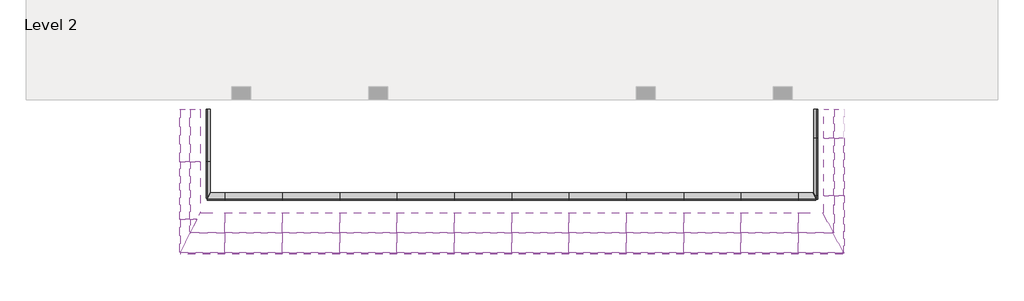
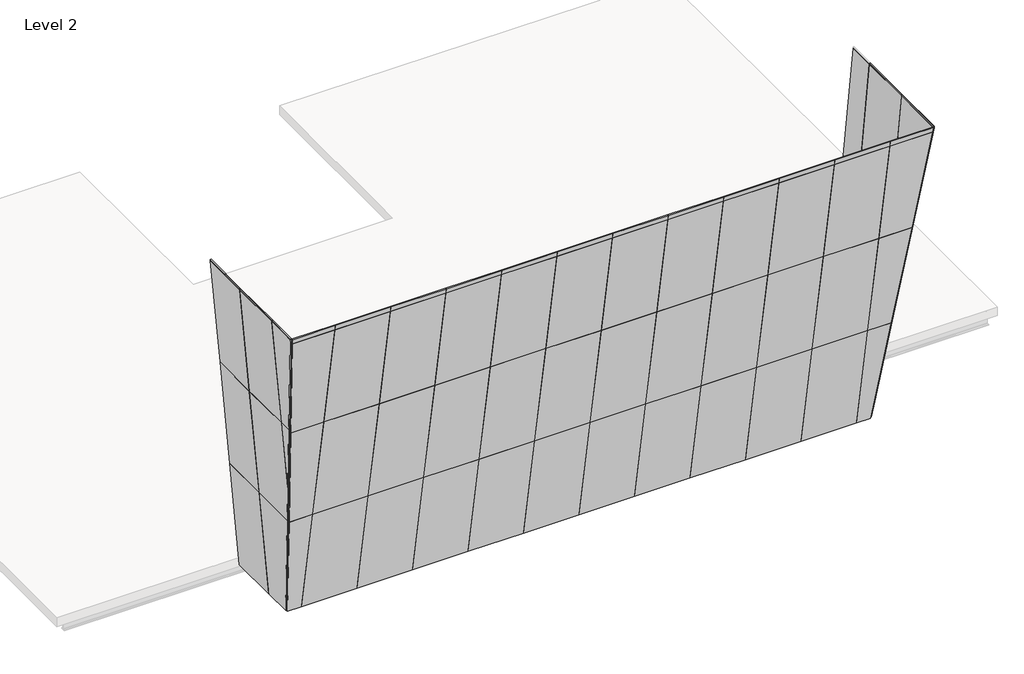
# One storey, part 1 of 2: 70 plates.
"""IFC4 building model written with IfcOpenShell, lengths in millimetres."""

import ifcopenshell
import ifcopenshell.guid

model = None  # the IFC model being written
_history = None  # IfcOwnerHistory: only IFC2X3 demands one
_inside = {}  # id of a spatial element -> (the spatial element, [elements in it])
_under = {}  # id of a project, library or spatial element -> (it, [spatial elements below it])
_declared = {}  # id of a project -> (the project, [libraries it declares])
_typed = {}  # id of a type object -> (the type object, [elements of that type])
_made_of = {}  # id of a material, layer set ... -> (it, [elements and type objects made of it])


def new_model(schema):
    """Start an empty IFC model of exactly this schema.

    Asked for "IFC4X3", IfcOpenShell would pick the latest addendum, in which some entities
    have other attributes; the version numbers below select the first issue.
    IFC2X3 requires an IfcOwnerHistory on every rooted entity: one is made here for all.
    """
    global model, _history
    if schema == "IFC4X3":
        model = ifcopenshell.file(schema_version=(4, 3, 0, 0))
    else:
        model = ifcopenshell.file(schema=schema)
    _inside.clear()
    _under.clear()
    _declared.clear()
    _typed.clear()
    _made_of.clear()
    _history = None
    if model.schema == "IFC2X3":
        org = make("IfcOrganization", Name="unknown")
        user = make(
            "IfcPersonAndOrganization",
            ThePerson=make("IfcPerson", FamilyName="unknown"),
            TheOrganization=org,
        )
        app = make(
            "IfcApplication",
            ApplicationDeveloper=org,
            Version="unknown",
            ApplicationFullName="unknown",
            ApplicationIdentifier="unknown",
        )
        _history = make(
            "IfcOwnerHistory",
            OwningUser=user,
            OwningApplication=app,
            ChangeAction="ADDED",
            CreationDate=0,
        )
    return model


def make(cls, **values):
    """One entity of the class cls with the attributes given. An attribute that is None is left unset."""
    return model.create_entity(
        cls, **{name: value for name, value in values.items() if value is not None}
    )


def rooted(cls, **values):
    """An entity with a GlobalId (a new one), such as an element, a storey or a relation."""
    return make(cls, GlobalId=ifcopenshell.guid.new(), OwnerHistory=_history, **values)


def si_unit(unit_type, name, prefix=None):
    """IfcSIUnit, for example si_unit("LENGTHUNIT", "METRE", prefix="MILLI")."""
    return make("IfcSIUnit", UnitType=unit_type, Prefix=prefix, Name=name)


def assignment(units):
    """IfcUnitAssignment: the units of a project."""
    return None if units is None else make("IfcUnitAssignment", Units=units)


def point(xyz):
    """IfcCartesianPoint."""
    return None if xyz is None else make("IfcCartesianPoint", Coordinates=xyz)


def direction(xyz):
    """IfcDirection."""
    return None if xyz is None else make("IfcDirection", DirectionRatios=xyz)


def frame(location, z_axis=None, x_axis=None):
    """IfcAxis2Placement3D, a coordinate frame: its origin and axes. An axis left out is left unset."""
    return make(
        "IfcAxis2Placement3D",
        Location=point(location),
        Axis=direction(z_axis),
        RefDirection=direction(x_axis),
    )


def origin():
    """The frame at (0, 0, 0) with its axes left unset."""
    return frame((0.0, 0.0, 0.0))


def origin_with_axes():
    """The frame at (0, 0, 0) with the z axis (0, 0, 1) and the x axis (1, 0, 0) written out."""
    return frame((0.0, 0.0, 0.0), z_axis=(0.0, 0.0, 1.0), x_axis=(1.0, 0.0, 0.0))


def place(relative_to, where):
    """IfcLocalPlacement: puts the frame where relative to a parent placement (None: the world)."""
    return make(
        "IfcLocalPlacement", PlacementRelTo=relative_to, RelativePlacement=where
    )


def context(
    kind, dimensions, precision=None, world=None, true_north=None, identifier=None
):
    """IfcGeometricRepresentationContext, for example the 3D "Model" context."""
    return make(
        "IfcGeometricRepresentationContext",
        ContextIdentifier=identifier,
        ContextType=kind,
        CoordinateSpaceDimension=dimensions,
        Precision=precision,
        WorldCoordinateSystem=world,
        TrueNorth=true_north,
    )


def project(units=None, contexts=None):
    """IfcProject with its units and contexts."""
    return rooted(
        "IfcProject",
        Name="project",
        RepresentationContexts=contexts,
        UnitsInContext=assignment(units),
    )


def spatial(cls, under=None, at=None, **own):
    """A site, building, storey or space (cls), placed at a placement, below another one or the project."""
    s = rooted(cls, ObjectPlacement=at, **own)
    if under is not None:
        _under.setdefault(under.id(), (under, []))[1].append(s)
    return s


def polyline(points):
    """IfcPolyline through the points."""
    return make("IfcPolyline", Points=[point(p) for p in points])


def outline(outer, holes=None, kind="AREA"):
    """IfcArbitraryClosedProfileDef: a profile drawn as a closed curve; with holes, ...WithVoids."""
    if holes is None:
        return make("IfcArbitraryClosedProfileDef", ProfileType=kind, OuterCurve=outer)
    return make(
        "IfcArbitraryProfileDefWithVoids",
        ProfileType=kind,
        OuterCurve=outer,
        InnerCurves=holes,
    )


def extrude(swept, where, along, depth):
    """IfcExtrudedAreaSolid: the profile swept, set in the frame where, extruded along a direction by depth."""
    return make(
        "IfcExtrudedAreaSolid",
        SweptArea=swept,
        Position=where,
        ExtrudedDirection=direction(along),
        Depth=depth,
    )


def shape(context_of_items, identifier, shape_type, items):
    """IfcShapeRepresentation: the items that make up one representation, for example the "Body"."""
    return make(
        "IfcShapeRepresentation",
        ContextOfItems=context_of_items,
        RepresentationIdentifier=identifier,
        RepresentationType=shape_type,
        Items=items,
    )


def source(mapping_origin, context_of_items, identifier, shape_type, items):
    """IfcRepresentationMap: a shape defined once, which mapped items show again and again."""
    return make(
        "IfcRepresentationMap",
        MappingOrigin=mapping_origin,
        MappedRepresentation=shape(context_of_items, identifier, shape_type, items),
    )


def transform(
    local_origin,
    x_axis=None,
    y_axis=None,
    z_axis=None,
    scale=None,
    scale2=None,
    scale3=None,
    uniform=True,
):
    """IfcCartesianTransformationOperator3D, or its non-uniform kind. x_axis, y_axis, z_axis: its Axis1, 2, 3."""
    if uniform:
        return make(
            "IfcCartesianTransformationOperator3D",
            Axis1=direction(x_axis),
            Axis2=direction(y_axis),
            LocalOrigin=point(local_origin),
            Scale=scale,
            Axis3=direction(z_axis),
        )
    return make(
        "IfcCartesianTransformationOperator3DnonUniform",
        Axis1=direction(x_axis),
        Axis2=direction(y_axis),
        LocalOrigin=point(local_origin),
        Scale=scale,
        Axis3=direction(z_axis),
        Scale2=scale2,
        Scale3=scale3,
    )


def mapped(mapping_source, mapping_target):
    """IfcMappedItem: shows the shape of a source again, moved by a transform."""
    return make(
        "IfcMappedItem", MappingSource=mapping_source, MappingTarget=mapping_target
    )


def made_of(thing, what):
    """Note that an element or type object is made of a material, layer set ...; save() writes the relation."""
    if what is not None:
        _made_of.setdefault(what.id(), (what, []))[1].append(thing)
    return thing


def element(
    cls,
    number,
    at=None,
    inside=None,
    cuts=None,
    type_object=None,
    material=None,
    context=None,
    identifier="Body",
    shape_type=None,
    held_by="IfcProductDefinitionShape",
    body=None,
    shapes=None,
    **own,
):
    """One element of the class cls, such as IfcWall. Its Tag is "e" and its number.

    at: its placement. inside: the storey or other place that contains it. cuts: it is an
    opening in that element (IfcRelVoidsElement). A single representation is given by context,
    identifier, shape_type and body (its items); several are given by shapes. held_by: the class
    of the entity that holds the representations. save() writes the other relations.
    """
    e = rooted(cls, Tag="e%d" % number, ObjectPlacement=at, **own)
    if body is not None:
        shapes = [shape(context, identifier, shape_type, body)]
    if shapes is not None:
        e.Representation = make(held_by, Representations=shapes)
    if inside is not None:
        _inside.setdefault(inside.id(), (inside, []))[1].append(e)
    if cuts is not None:
        rooted(
            "IfcRelVoidsElement", RelatingBuildingElement=cuts, RelatedOpeningElement=e
        )
    if type_object is not None:
        _typed.setdefault(type_object.id(), (type_object, []))[1].append(e)
    return made_of(e, material)


def aggregate(whole, parts):
    """IfcRelAggregates: a whole, such as a stair, and the parts it consists of."""
    return rooted("IfcRelAggregates", RelatingObject=whole, RelatedObjects=parts)


def save(model, path):
    """Write the relations noted so far, then the file.

    IfcRelAggregates (storeys below a building ...), IfcRelContainedInSpatialStructure (elements
    in a storey), IfcRelDefinesByType, IfcRelAssociatesMaterial and IfcRelDeclares: one each for
    every whole, place, type object, material and project.
    """
    for whole, parts in _under.values():
        aggregate(whole, parts)
    for where, things in _inside.values():
        rooted(
            "IfcRelContainedInSpatialStructure",
            RelatedElements=things,
            RelatingStructure=where,
        )
    for kind, things in _typed.values():
        rooted("IfcRelDefinesByType", RelatedObjects=things, RelatingType=kind)
    for what, things in _made_of.values():
        rooted("IfcRelAssociatesMaterial", RelatedObjects=things, RelatingMaterial=what)
    for by, libraries in _declared.values():
        rooted("IfcRelDeclares", RelatingContext=by, RelatedDefinitions=libraries)
    model.write(path)


def system_panel_glazed_2e91cb65(model_context):
    return source(origin(), model_context, "Body", "SweptSolid", [
        extrude(outline(polyline([(838.2000002, -44.45), (-838.2000002, -44.45), (-838.2000002, -19.05), (838.2000002, -19.05), (838.2000002, -44.45)])), origin_with_axes(), (0.0, 0.0, 1.0), 3657.6),
    ])


def system_panel_glazed_41c8569a(model_context):
    return source(origin(), model_context, "Body", "SweptSolid", [
        extrude(outline(polyline([(3054.1438606, -268.2393521), (0.0, 268.2393521), (3054.1438606, 268.2393521), (3054.1438606, -268.2393521)])), frame((0.0, -44.45, 0.0), z_axis=(0.0, 1.0, 0.0), x_axis=(0.0, 0.0, 1.0)), (0.0, 0.0, 1.0), 25.4),
    ])


def system_panel_glazed_2bad594a(model_context):
    return source(origin(), model_context, "Body", "SweptSolid", [
        extrude(outline(polyline([(0.0, -797.3917397), (0.0, 154.912342), (3657.6, 797.3917397), (3657.6, -797.3917397), (0.0, -797.3917397)])), frame((0.0, -44.45, 0.0), z_axis=(0.0, 1.0, 0.0), x_axis=(0.0, 0.0, 1.0)), (0.0, 0.0, 1.0), 25.4),
    ])


def system_panel_glazed_87679f4c(model_context):
    return source(origin(), model_context, "Body", "SweptSolid", [
        extrude(outline(polyline([(0.0, -914.4), (0.0, 680.3834794), (1332.2432262, 914.4), (3657.6, 914.4), (3657.6, -914.4), (0.0, -914.4)])), frame((0.0, -44.45, 0.0), z_axis=(0.0, 1.0, 0.0), x_axis=(0.0, 0.0, 1.0)), (0.0, 0.0, 1.0), 25.4),
    ])


def system_panel_glazed_96c5221b(model_context):
    return source(origin(), model_context, "Body", "SweptSolid", [
        extrude(outline(polyline([(0.0, -204.2314386), (2325.3567738, 204.2314386), (2325.3567738, -204.2314386), (0.0, -204.2314386)])), frame((0.0, -44.45, 0.0), z_axis=(0.0, 1.0, 0.0), x_axis=(0.0, 0.0, 1.0)), (0.0, 0.0, 1.0), 25.4),
    ])


def system_panel_glazed_1f34555f(model_context):
    return source(origin(), model_context, "Body", "SweptSolid", [
        extrude(outline(polyline([(914.4, -44.45), (-914.4, -44.45), (-914.4, -19.05), (914.4, -19.05), (914.4, -44.45)])), origin_with_axes(), (0.0, 0.0, 1.0), 3657.6),
    ])


def system_panel_glazed_ce152239(model_context):
    return source(origin(), model_context, "Body", "SweptSolid", [
        extrude(outline(polyline([(0.0, -525.4711374), (0.0, -117.0082603), (3657.6, 525.4711374), (3657.6, -525.4711374), (0.0, -525.4711374)])), frame((0.0, -44.45, 0.0), z_axis=(0.0, 1.0, 0.0), x_axis=(0.0, 0.0, 1.0)), (0.0, 0.0, 1.0), 25.4),
    ])


def system_panel_glazed_8b4ddac8(model_context):
    return source(origin(), model_context, "Body", "SweptSolid", [
        extrude(outline(polyline([(838.2000002, -44.45), (-838.2000002, -44.45), (-838.2000002, -19.05), (838.2000002, -19.05), (838.2000002, -44.45)])), origin_with_axes(), (0.0, 0.0, 1.0), 41.9143134),
    ])


def system_panel_glazed_7f82afe2(model_context):
    return source(origin(), model_context, "Body", "SweptSolid", [
        extrude(outline(polyline([(914.4, -44.45), (-914.4, -44.45), (-914.4, -19.05), (914.4, -19.05), (914.4, -44.45)])), origin_with_axes(), (0.0, 0.0, 1.0), 41.9143134),
    ])


def system_panel_glazed_3146f186(model_context):
    return source(origin(), model_context, "Body", "SweptSolid", [
        extrude(outline(polyline([(0.0, -529.1523878), (0.0, 521.789887), (41.9143134, 529.1523878), (41.9143134, -529.1523878), (0.0, -529.1523878)])), frame((0.0, -44.45, 0.0), z_axis=(0.0, 1.0, 0.0), x_axis=(0.0, 0.0, 1.0)), (0.0, 0.0, 1.0), 25.4),
    ])


def system_panel_glazed_f4345ae3(model_context):
    return source(origin(), model_context, "Body", "SweptSolid", [
        extrude(outline(polyline([(914.4, -44.45), (-914.4, -44.45), (-914.4, -19.05), (914.4, -19.05), (914.4, -44.45)])), origin_with_axes(), (0.0, 0.0, 1.0), 169.2731269),
    ])


def system_panel_glazed_866ab655(model_context):
    return source(origin(), model_context, "Body", "SweptSolid", [
        extrude(outline(polyline([(0.0, -808.3993064), (0.0, 914.4), (3657.6, 914.4), (3657.6, -914.4), (603.4561394, -914.4), (0.0, -808.3993064)])), frame((0.0, -44.45, 0.0), z_axis=(0.0, 1.0, 0.0), x_axis=(0.0, 0.0, 1.0)), (0.0, 0.0, 1.0), 25.4),
    ])


def system_panel_glazed_b062bbc2(model_context):
    return source(origin(), model_context, "Body", "SweptSolid", [
        extrude(outline(polyline([(465.8483058, -44.45), (-465.8483058, -44.45), (-465.8483058, -19.05), (465.8483058, -19.05), (465.8483058, -44.45)])), origin_with_axes(), (0.0, 0.0, 1.0), 3657.6),
    ])


def system_panel_glazed_bcd6892e(model_context):
    return source(origin(), model_context, "Body", "SweptSolid", [
        extrude(outline(polyline([(0.0, 53.0003468), (0.0, 589.4790509), (3657.6, 589.4790509), (3657.6, -589.4790509), (0.0, 53.0003468)])), frame((0.0, -44.45, 0.0), z_axis=(0.0, 1.0, 0.0), x_axis=(0.0, 0.0, 1.0)), (0.0, 0.0, 1.0), 25.4),
    ])


def system_panel_glazed_e7bd2299(model_context):
    return source(origin(), model_context, "Body", "SweptSolid", [
        extrude(outline(polyline([(0.0, -268.2393521), (0.0, 910.7187498), (3657.6, 910.7187498), (3657.6, -910.7187498), (0.0, -268.2393521)])), frame((0.0, -44.45, 0.0), z_axis=(0.0, 1.0, 0.0), x_axis=(0.0, 0.0, 1.0)), (0.0, 0.0, 1.0), 25.4),
    ])


def system_panel_glazed_0a43eb3e(model_context):
    return source(origin(), model_context, "Body", "SweptSolid", [
        extrude(outline(polyline([(0.0, -907.0374994), (0.0, 914.4000002), (41.9143134, 914.4000002), (41.9143134, -914.4000002), (0.0, -907.0374994)])), frame((0.0, -44.45, 0.0), z_axis=(0.0, 1.0, 0.0), x_axis=(0.0, 0.0, 1.0)), (0.0, 0.0, 1.0), 25.4),
    ])


def system_panel_glazed_35afb83b(model_context):
    return source(origin(), model_context, "Body", "SweptSolid", [
        extrude(outline(polyline([(0.0, -71.0314805), (0.0, 386.1685195), (3657.6, 386.1685195), (3657.6, -386.1685195), (0.0, -71.0314805)])), frame((0.0, -44.45, 0.0), z_axis=(0.0, 1.0, 0.0), x_axis=(0.0, 0.0, 1.0)), (0.0, 0.0, 1.0), 25.4),
    ])


def system_panel_glazed_ca25d662(model_context):
    return source(origin(), model_context, "Body", "SweptSolid", [
        extrude(outline(polyline([(0.0, -386.1685195), (0.0, 71.0314805), (3657.6, 386.1685195), (3657.6, -386.1685195), (0.0, -386.1685195)])), frame((0.0, -44.45, 0.0), z_axis=(0.0, 1.0, 0.0), x_axis=(0.0, 0.0, 1.0)), (0.0, 0.0, 1.0), 25.4),
    ])


def system_panel_glazed_d5b9b34d(model_context):
    return source(origin(), model_context, "Body", "SweptSolid", [
        extrude(outline(polyline([(0.0, -228.6), (0.0, 543.7370389), (3657.6, 543.7370389), (3657.6, -543.7370389), (0.0, -228.6)])), frame((0.0, -44.45, 0.0), z_axis=(0.0, 1.0, 0.0), x_axis=(0.0, 0.0, 1.0)), (0.0, 0.0, 1.0), 25.4),
    ])


def system_panel_glazed_127879aa(model_context):
    return source(origin(), model_context, "Body", "SweptSolid", [
        extrude(outline(polyline([(0.0, -543.7370389), (0.0, 228.6), (3657.6, 543.7370389), (3657.6, -543.7370389), (0.0, -543.7370389)])), frame((0.0, -44.45, 0.0), z_axis=(0.0, 1.0, 0.0), x_axis=(0.0, 0.0, 1.0)), (0.0, 0.0, 1.0), 25.4),
    ])


def system_panel_glazed_cde5e94a(model_context):
    return source(origin(), model_context, "Body", "SweptSolid", [
        extrude(outline(polyline([(0.0, -386.1685195), (0.0, 701.3055584), (3657.6, 701.3055584), (3657.6, -701.3055584), (0.0, -386.1685195)])), frame((0.0, -44.45, 0.0), z_axis=(0.0, 1.0, 0.0), x_axis=(0.0, 0.0, 1.0)), (0.0, 0.0, 1.0), 25.4),
    ])


def system_panel_glazed_b3fa7013(model_context):
    return source(origin(), model_context, "Body", "SweptSolid", [
        extrude(outline(polyline([(0.0, -701.3055584), (0.0, 386.1685195), (3657.6, 701.3055584), (3657.6, -701.3055584), (0.0, -701.3055584)])), frame((0.0, -44.45, 0.0), z_axis=(0.0, 1.0, 0.0), x_axis=(0.0, 0.0, 1.0)), (0.0, 0.0, 1.0), 25.4),
    ])


def system_panel_glazed_d86b06c2(model_context):
    return source(origin(), model_context, "Body", "SweptSolid", [
        extrude(outline(polyline([(0.0, -694.0133132), (0.0, 708.5978036), (169.2731269, 708.5978036), (169.2731269, -708.5978036), (0.0, -694.0133132)])), frame((0.0, -44.45, 0.0), z_axis=(0.0, 1.0, 0.0), x_axis=(0.0, 0.0, 1.0)), (0.0, 0.0, 1.0), 25.4),
    ])


def system_panel_glazed_9c30f1a4(model_context):
    return source(origin(), model_context, "Body", "SweptSolid", [
        extrude(outline(polyline([(0.0, -708.5978036), (0.0, 694.0133132), (169.2731269, 708.5978036), (169.2731269, -708.5978036), (0.0, -708.5978036)])), frame((0.0, -44.45, 0.0), z_axis=(0.0, 1.0, 0.0), x_axis=(0.0, 0.0, 1.0)), (0.0, 0.0, 1.0), 25.4),
    ])


model = new_model("IFC4")

# Units and contexts
model_context = context("Model", 3, world=origin())
ifc_project = project(units=[si_unit("LENGTHUNIT", "METRE", prefix="MILLI")], contexts=[model_context])

# Site, building, storey
site = spatial("IfcSite", under=ifc_project)
building = spatial("IfcBuilding", under=site)
storey = spatial("IfcBuildingStorey", under=building, Name="Level 2", Elevation=3657.6)

# Plates
placement = place(None, origin())
system_panel_glazed_shape = system_panel_glazed_2e91cb65(model_context)
element("IfcPlate", 1, ObjectType="System Panel : Glazed", at=placement, inside=storey, context=model_context, shape_type="MappedRepresentation", body=[
    mapped(system_panel_glazed_shape, transform((-10766.9154339, -10749.0984697, 3656.4931221), x_axis=(0.0, -1.0, 0.0), y_axis=(0.9961946980917455, 0.0, 0.08715574274765803), z_axis=(-0.08715574274765803, 0.0, 0.9961946980917455))),
])
element("IfcPlate", 2, ObjectType="System Panel : Glazed", at=placement, inside=storey, context=model_context, shape_type="MappedRepresentation", body=[
    mapped(system_panel_glazed_shape, transform((-11085.6962786, -10749.0984697, 7300.1748498), x_axis=(0.0, -1.0, 0.0), y_axis=(0.9961946980917455, 0.0, 0.08715574274765803), z_axis=(-0.08715574274765803, 0.0, 0.9961946980917455))),
])
element("IfcPlate", 3, ObjectType="System Panel : Glazed", at=placement, inside=storey, context=model_context, shape_type="MappedRepresentation", body=[
    mapped(system_panel_glazed_shape, transform((-11404.4771233, -10749.0984697, 10943.8565775), x_axis=(0.0, -1.0, 0.0), y_axis=(0.9961946980917455, 0.0, 0.08715574274765803), z_axis=(-0.08715574274765803, 0.0, 0.9961946980917455))),
])
system_panel_glazed_2_shape = system_panel_glazed_41c8569a(model_context)
element("IfcPlate", 4, ObjectType="System Panel : Glazed", at=placement, inside=storey, context=model_context, shape_type="MappedRepresentation", body=[
    mapped(system_panel_glazed_2_shape, transform((8487.8855556, -12939.6344332, 4257.6529286), x_axis=(0.0, 1.0, 0.0), y_axis=(-0.9961946980917455, 0.0, 0.08715574274765803), z_axis=(0.08715574274765803, 0.0, 0.9961946980917455))),
])
system_panel_glazed_3_shape = system_panel_glazed_2bad594a(model_context)
element("IfcPlate", 5, ObjectType="System Panel : Glazed", at=placement, inside=storey, context=model_context, shape_type="MappedRepresentation", body=[
    mapped(system_panel_glazed_3_shape, transform((-10766.9154339, -12384.6902096, 3656.4931221), x_axis=(0.0, -1.0, 0.0), y_axis=(0.9961946980917455, 0.0, 0.08715574274765803), z_axis=(-0.08715574274765803, 0.0, 0.9961946980917455))),
])
system_panel_glazed_4_shape = system_panel_glazed_87679f4c(model_context)
element("IfcPlate", 6, ObjectType="System Panel : Glazed", at=placement, inside=storey, context=model_context, shape_type="MappedRepresentation", body=[
    mapped(system_panel_glazed_4_shape, transform((-11085.6962786, -12501.6984699, 7300.1748498), x_axis=(0.0, -1.0, 0.0), y_axis=(0.9961946980917455, 0.0, 0.08715574274765803), z_axis=(-0.08715574274765803, 0.0, 0.9961946980917455))),
])
system_panel_glazed_5_shape = system_panel_glazed_96c5221b(model_context)
element("IfcPlate", 7, ObjectType="System Panel : Glazed", at=placement, inside=storey, context=model_context, shape_type="MappedRepresentation", body=[
    mapped(system_panel_glazed_5_shape, transform((-11201.8089265, -13620.3299085, 8627.3484884), x_axis=(0.0, -1.0, 0.0), y_axis=(0.9961946980917455, 0.0, 0.08715574274765803), z_axis=(-0.08715574274765803, 0.0, 0.9961946980917455))),
])
system_panel_glazed_6_shape = system_panel_glazed_1f34555f(model_context)
element("IfcPlate", 8, ObjectType="System Panel : Glazed", at=placement, inside=storey, context=model_context, shape_type="MappedRepresentation", body=[
    mapped(system_panel_glazed_6_shape, transform((-11404.4771233, -12501.6984699, 10943.8565775), x_axis=(0.0, -1.0, 0.0), y_axis=(0.9961946980917455, 0.0, 0.08715574274765803), z_axis=(-0.08715574274765803, 0.0, 0.9961946980917455))),
])
element("IfcPlate", 9, ObjectType="System Panel : Glazed", at=placement, inside=storey, context=model_context, shape_type="MappedRepresentation", body=[
    mapped(system_panel_glazed_6_shape, transform((-9408.1607851, -12552.1096101, 3655.3946681), x_axis=(1.0, 0.0, 0.0), y_axis=(0.0, 0.9848077530122081, 0.17364817766693014), z_axis=(0.0, -0.17364817766693014, 0.9848077530122081))),
])
element("IfcPlate", 10, ObjectType="System Panel : Glazed", at=placement, inside=storey, context=model_context, shape_type="MappedRepresentation", body=[
    mapped(system_panel_glazed_6_shape, transform((-7579.3607851, -12552.1096101, 3655.3946681), x_axis=(1.0, 0.0, 0.0), y_axis=(0.0, 0.9848077530122081, 0.17364817766693014), z_axis=(0.0, -0.17364817766693014, 0.9848077530122081))),
])
element("IfcPlate", 11, ObjectType="System Panel : Glazed", at=placement, inside=storey, context=model_context, shape_type="MappedRepresentation", body=[
    mapped(system_panel_glazed_6_shape, transform((-5750.5607851, -12552.1096101, 3655.3946681), x_axis=(1.0, 0.0, 0.0), y_axis=(0.0, 0.9848077530122081, 0.17364817766693014), z_axis=(0.0, -0.17364817766693014, 0.9848077530122081))),
])
element("IfcPlate", 12, ObjectType="System Panel : Glazed", at=placement, inside=storey, context=model_context, shape_type="MappedRepresentation", body=[
    mapped(system_panel_glazed_6_shape, transform((-3921.7607851, -12552.1096101, 3655.3946681), x_axis=(1.0, 0.0, 0.0), y_axis=(0.0, 0.9848077530122081, 0.17364817766693014), z_axis=(0.0, -0.17364817766693014, 0.9848077530122081))),
])
element("IfcPlate", 13, ObjectType="System Panel : Glazed", at=placement, inside=storey, context=model_context, shape_type="MappedRepresentation", body=[
    mapped(system_panel_glazed_6_shape, transform((-2092.9607851, -12552.1096101, 3655.3946681), x_axis=(1.0, 0.0, 0.0), y_axis=(0.0, 0.9848077530122081, 0.17364817766693014), z_axis=(0.0, -0.17364817766693014, 0.9848077530122081))),
])
element("IfcPlate", 14, ObjectType="System Panel : Glazed", at=placement, inside=storey, context=model_context, shape_type="MappedRepresentation", body=[
    mapped(system_panel_glazed_6_shape, transform((-264.1607851, -12552.1096101, 3655.3946681), x_axis=(1.0, 0.0, 0.0), y_axis=(0.0, 0.9848077530122081, 0.17364817766693014), z_axis=(0.0, -0.17364817766693014, 0.9848077530122081))),
])
element("IfcPlate", 15, ObjectType="System Panel : Glazed", at=placement, inside=storey, context=model_context, shape_type="MappedRepresentation", body=[
    mapped(system_panel_glazed_6_shape, transform((1564.6392149, -12552.1096101, 3655.3946681), x_axis=(1.0, 0.0, 0.0), y_axis=(0.0, 0.9848077530122081, 0.17364817766693014), z_axis=(0.0, -0.17364817766693014, 0.9848077530122081))),
])
element("IfcPlate", 16, ObjectType="System Panel : Glazed", at=placement, inside=storey, context=model_context, shape_type="MappedRepresentation", body=[
    mapped(system_panel_glazed_6_shape, transform((3393.4392149, -12552.1096101, 3655.3946681), x_axis=(1.0, 0.0, 0.0), y_axis=(0.0, 0.9848077530122081, 0.17364817766693014), z_axis=(0.0, -0.17364817766693014, 0.9848077530122081))),
])
element("IfcPlate", 17, ObjectType="System Panel : Glazed", at=placement, inside=storey, context=model_context, shape_type="MappedRepresentation", body=[
    mapped(system_panel_glazed_6_shape, transform((5222.2392149, -12552.1096101, 3655.3946681), x_axis=(1.0, 0.0, 0.0), y_axis=(0.0, 0.9848077530122081, 0.17364817766693014), z_axis=(0.0, -0.17364817766693014, 0.9848077530122081))),
])
element("IfcPlate", 18, ObjectType="System Panel : Glazed", at=placement, inside=storey, context=model_context, shape_type="MappedRepresentation", body=[
    mapped(system_panel_glazed_6_shape, transform((7051.0392149, -12552.1096101, 3655.3946681), x_axis=(1.0, 0.0, 0.0), y_axis=(0.0, 0.9848077530122081, 0.17364817766693014), z_axis=(0.0, -0.17364817766693014, 0.9848077530122081))),
])
element("IfcPlate", 19, ObjectType="System Panel : Glazed", at=placement, inside=storey, context=model_context, shape_type="MappedRepresentation", body=[
    mapped(system_panel_glazed_6_shape, transform((-9408.1607851, -13187.2451847, 7257.4275056), x_axis=(1.0, 0.0, 0.0), y_axis=(0.0, 0.9848077530122081, 0.17364817766693014), z_axis=(0.0, -0.17364817766693014, 0.9848077530122081))),
])
element("IfcPlate", 20, ObjectType="System Panel : Glazed", at=placement, inside=storey, context=model_context, shape_type="MappedRepresentation", body=[
    mapped(system_panel_glazed_6_shape, transform((-7579.3607851, -13187.2451847, 7257.4275056), x_axis=(1.0, 0.0, 0.0), y_axis=(0.0, 0.9848077530122081, 0.17364817766693014), z_axis=(0.0, -0.17364817766693014, 0.9848077530122081))),
])
element("IfcPlate", 21, ObjectType="System Panel : Glazed", at=placement, inside=storey, context=model_context, shape_type="MappedRepresentation", body=[
    mapped(system_panel_glazed_6_shape, transform((-5750.5607851, -13187.2451847, 7257.4275056), x_axis=(1.0, 0.0, 0.0), y_axis=(0.0, 0.9848077530122081, 0.17364817766693014), z_axis=(0.0, -0.17364817766693014, 0.9848077530122081))),
])
element("IfcPlate", 22, ObjectType="System Panel : Glazed", at=placement, inside=storey, context=model_context, shape_type="MappedRepresentation", body=[
    mapped(system_panel_glazed_6_shape, transform((-3921.7607851, -13187.2451847, 7257.4275056), x_axis=(1.0, 0.0, 0.0), y_axis=(0.0, 0.9848077530122081, 0.17364817766693014), z_axis=(0.0, -0.17364817766693014, 0.9848077530122081))),
])
element("IfcPlate", 23, ObjectType="System Panel : Glazed", at=placement, inside=storey, context=model_context, shape_type="MappedRepresentation", body=[
    mapped(system_panel_glazed_6_shape, transform((-2092.9607851, -13187.2451847, 7257.4275056), x_axis=(1.0, 0.0, 0.0), y_axis=(0.0, 0.9848077530122081, 0.17364817766693014), z_axis=(0.0, -0.17364817766693014, 0.9848077530122081))),
])
element("IfcPlate", 24, ObjectType="System Panel : Glazed", at=placement, inside=storey, context=model_context, shape_type="MappedRepresentation", body=[
    mapped(system_panel_glazed_6_shape, transform((-264.1607851, -13187.2451847, 7257.4275056), x_axis=(1.0, 0.0, 0.0), y_axis=(0.0, 0.9848077530122081, 0.17364817766693014), z_axis=(0.0, -0.17364817766693014, 0.9848077530122081))),
])
element("IfcPlate", 25, ObjectType="System Panel : Glazed", at=placement, inside=storey, context=model_context, shape_type="MappedRepresentation", body=[
    mapped(system_panel_glazed_6_shape, transform((1564.6392149, -13187.2451847, 7257.4275056), x_axis=(1.0, 0.0, 0.0), y_axis=(0.0, 0.9848077530122081, 0.17364817766693014), z_axis=(0.0, -0.17364817766693014, 0.9848077530122081))),
])
element("IfcPlate", 26, ObjectType="System Panel : Glazed", at=placement, inside=storey, context=model_context, shape_type="MappedRepresentation", body=[
    mapped(system_panel_glazed_6_shape, transform((3393.4392149, -13187.2451847, 7257.4275056), x_axis=(1.0, 0.0, 0.0), y_axis=(0.0, 0.9848077530122081, 0.17364817766693014), z_axis=(0.0, -0.17364817766693014, 0.9848077530122081))),
])
element("IfcPlate", 27, ObjectType="System Panel : Glazed", at=placement, inside=storey, context=model_context, shape_type="MappedRepresentation", body=[
    mapped(system_panel_glazed_6_shape, transform((5222.2392149, -13187.2451847, 7257.4275056), x_axis=(1.0, 0.0, 0.0), y_axis=(0.0, 0.9848077530122081, 0.17364817766693014), z_axis=(0.0, -0.17364817766693014, 0.9848077530122081))),
])
element("IfcPlate", 28, ObjectType="System Panel : Glazed", at=placement, inside=storey, context=model_context, shape_type="MappedRepresentation", body=[
    mapped(system_panel_glazed_6_shape, transform((7051.0392149, -13187.2451847, 7257.4275056), x_axis=(1.0, 0.0, 0.0), y_axis=(0.0, 0.9848077530122081, 0.17364817766693014), z_axis=(0.0, -0.17364817766693014, 0.9848077530122081))),
])
element("IfcPlate", 29, ObjectType="System Panel : Glazed", at=placement, inside=storey, context=model_context, shape_type="MappedRepresentation", body=[
    mapped(system_panel_glazed_6_shape, transform((-9408.1607851, -13822.3807593, 10859.460343), x_axis=(1.0, 0.0, 0.0), y_axis=(0.0, 0.9848077530122081, 0.17364817766693014), z_axis=(0.0, -0.17364817766693014, 0.9848077530122081))),
])
element("IfcPlate", 30, ObjectType="System Panel : Glazed", at=placement, inside=storey, context=model_context, shape_type="MappedRepresentation", body=[
    mapped(system_panel_glazed_6_shape, transform((-7579.3607851, -13822.3807593, 10859.460343), x_axis=(1.0, 0.0, 0.0), y_axis=(0.0, 0.9848077530122081, 0.17364817766693014), z_axis=(0.0, -0.17364817766693014, 0.9848077530122081))),
])
element("IfcPlate", 31, ObjectType="System Panel : Glazed", at=placement, inside=storey, context=model_context, shape_type="MappedRepresentation", body=[
    mapped(system_panel_glazed_6_shape, transform((-5750.5607851, -13822.3807593, 10859.460343), x_axis=(1.0, 0.0, 0.0), y_axis=(0.0, 0.9848077530122081, 0.17364817766693014), z_axis=(0.0, -0.17364817766693014, 0.9848077530122081))),
])
element("IfcPlate", 32, ObjectType="System Panel : Glazed", at=placement, inside=storey, context=model_context, shape_type="MappedRepresentation", body=[
    mapped(system_panel_glazed_6_shape, transform((-3921.7607851, -13822.3807593, 10859.460343), x_axis=(1.0, 0.0, 0.0), y_axis=(0.0, 0.9848077530122081, 0.17364817766693014), z_axis=(0.0, -0.17364817766693014, 0.9848077530122081))),
])
element("IfcPlate", 33, ObjectType="System Panel : Glazed", at=placement, inside=storey, context=model_context, shape_type="MappedRepresentation", body=[
    mapped(system_panel_glazed_6_shape, transform((-2092.9607851, -13822.3807593, 10859.460343), x_axis=(1.0, 0.0, 0.0), y_axis=(0.0, 0.9848077530122081, 0.17364817766693014), z_axis=(0.0, -0.17364817766693014, 0.9848077530122081))),
])
element("IfcPlate", 34, ObjectType="System Panel : Glazed", at=placement, inside=storey, context=model_context, shape_type="MappedRepresentation", body=[
    mapped(system_panel_glazed_6_shape, transform((-264.1607851, -13822.3807593, 10859.460343), x_axis=(1.0, 0.0, 0.0), y_axis=(0.0, 0.9848077530122081, 0.17364817766693014), z_axis=(0.0, -0.17364817766693014, 0.9848077530122081))),
])
element("IfcPlate", 35, ObjectType="System Panel : Glazed", at=placement, inside=storey, context=model_context, shape_type="MappedRepresentation", body=[
    mapped(system_panel_glazed_6_shape, transform((1564.6392149, -13822.3807593, 10859.460343), x_axis=(1.0, 0.0, 0.0), y_axis=(0.0, 0.9848077530122081, 0.17364817766693014), z_axis=(0.0, -0.17364817766693014, 0.9848077530122081))),
])
element("IfcPlate", 36, ObjectType="System Panel : Glazed", at=placement, inside=storey, context=model_context, shape_type="MappedRepresentation", body=[
    mapped(system_panel_glazed_6_shape, transform((3393.4392149, -13822.3807593, 10859.460343), x_axis=(1.0, 0.0, 0.0), y_axis=(0.0, 0.9848077530122081, 0.17364817766693014), z_axis=(0.0, -0.17364817766693014, 0.9848077530122081))),
])
element("IfcPlate", 37, ObjectType="System Panel : Glazed", at=placement, inside=storey, context=model_context, shape_type="MappedRepresentation", body=[
    mapped(system_panel_glazed_6_shape, transform((5222.2392149, -13822.3807593, 10859.460343), x_axis=(1.0, 0.0, 0.0), y_axis=(0.0, 0.9848077530122081, 0.17364817766693014), z_axis=(0.0, -0.17364817766693014, 0.9848077530122081))),
])
element("IfcPlate", 38, ObjectType="System Panel : Glazed", at=placement, inside=storey, context=model_context, shape_type="MappedRepresentation", body=[
    mapped(system_panel_glazed_6_shape, transform((7051.0392149, -13822.3807593, 10859.460343), x_axis=(1.0, 0.0, 0.0), y_axis=(0.0, 0.9848077530122081, 0.17364817766693014), z_axis=(0.0, -0.17364817766693014, 0.9848077530122081))),
])
element("IfcPlate", 39, ObjectType="System Panel : Glazed", at=placement, inside=storey, context=model_context, shape_type="MappedRepresentation", body=[
    mapped(system_panel_glazed_6_shape, transform((8754.0717322, -11756.9950812, 7300.1748498), x_axis=(0.0, 1.0, 0.0), y_axis=(-0.9961946980917455, 0.0, 0.08715574274765803), z_axis=(0.08715574274765803, 0.0, 0.9961946980917455))),
])
element("IfcPlate", 40, ObjectType="System Panel : Glazed", at=placement, inside=storey, context=model_context, shape_type="MappedRepresentation", body=[
    mapped(system_panel_glazed_6_shape, transform((9072.8525769, -11756.9950812, 10943.8565775), x_axis=(0.0, 1.0, 0.0), y_axis=(-0.9961946980917455, 0.0, 0.08715574274765803), z_axis=(0.08715574274765803, 0.0, 0.9961946980917455))),
])
system_panel_glazed_7_shape = system_panel_glazed_ce152239(model_context)
element("IfcPlate", 41, ObjectType="System Panel : Glazed", at=placement, inside=storey, context=model_context, shape_type="MappedRepresentation", body=[
    mapped(system_panel_glazed_7_shape, transform((-11404.4771233, -13941.5696073, 10943.8565775), x_axis=(0.0, -1.0, 0.0), y_axis=(0.9961946980917455, 0.0, 0.08715574274765803), z_axis=(-0.08715574274765803, 0.0, 0.9961946980917455))),
])
system_panel_glazed_8_shape = system_panel_glazed_8b4ddac8(model_context)
element("IfcPlate", 42, ObjectType="System Panel : Glazed", at=placement, inside=storey, context=model_context, shape_type="MappedRepresentation", body=[
    mapped(system_panel_glazed_8_shape, transform((-11723.2579679, -10749.0984697, 14587.5383053), x_axis=(0.0, -1.0, 0.0), y_axis=(0.9961946980917455, 0.0, 0.08715574274765803), z_axis=(-0.08715574274765803, 0.0, 0.9961946980917455))),
])
system_panel_glazed_9_shape = system_panel_glazed_7f82afe2(model_context)
element("IfcPlate", 43, ObjectType="System Panel : Glazed", at=placement, inside=storey, context=model_context, shape_type="MappedRepresentation", body=[
    mapped(system_panel_glazed_9_shape, transform((-11723.2579679, -12501.6984699, 14587.5383053), x_axis=(0.0, -1.0, 0.0), y_axis=(0.9961946980917455, 0.0, 0.08715574274765803), z_axis=(-0.08715574274765803, 0.0, 0.9961946980917455))),
])
element("IfcPlate", 44, ObjectType="System Panel : Glazed", at=placement, inside=storey, context=model_context, shape_type="MappedRepresentation", body=[
    mapped(system_panel_glazed_9_shape, transform((9391.6334216, -11756.9950812, 14587.5383053), x_axis=(0.0, 1.0, 0.0), y_axis=(-0.9961946980917455, 0.0, 0.08715574274765803), z_axis=(0.08715574274765803, 0.0, 0.9961946980917455))),
])
system_panel_glazed_10_shape = system_panel_glazed_3146f186(model_context)
element("IfcPlate", 45, ObjectType="System Panel : Glazed", at=placement, inside=storey, context=model_context, shape_type="MappedRepresentation", body=[
    mapped(system_panel_glazed_10_shape, transform((-11723.2579679, -13945.2508577, 14587.5383053), x_axis=(0.0, -1.0, 0.0), y_axis=(0.9961946980917455, 0.0, 0.08715574274765803), z_axis=(-0.08715574274765803, 0.0, 0.9961946980917455))),
])
system_panel_glazed_11_shape = system_panel_glazed_f4345ae3(model_context)
element("IfcPlate", 46, ObjectType="System Panel : Glazed", at=placement, inside=storey, context=model_context, shape_type="MappedRepresentation", body=[
    mapped(system_panel_glazed_11_shape, transform((-9408.1607851, -14457.516334, 14461.4931804), x_axis=(1.0, 0.0, 0.0), y_axis=(0.0, 0.9848077530122081, 0.17364817766693014), z_axis=(0.0, -0.17364817766693014, 0.9848077530122081))),
])
element("IfcPlate", 47, ObjectType="System Panel : Glazed", at=placement, inside=storey, context=model_context, shape_type="MappedRepresentation", body=[
    mapped(system_panel_glazed_11_shape, transform((-7579.3607851, -14457.516334, 14461.4931804), x_axis=(1.0, 0.0, 0.0), y_axis=(0.0, 0.9848077530122081, 0.17364817766693014), z_axis=(0.0, -0.17364817766693014, 0.9848077530122081))),
])
element("IfcPlate", 48, ObjectType="System Panel : Glazed", at=placement, inside=storey, context=model_context, shape_type="MappedRepresentation", body=[
    mapped(system_panel_glazed_11_shape, transform((-5750.5607851, -14457.516334, 14461.4931804), x_axis=(1.0, 0.0, 0.0), y_axis=(0.0, 0.9848077530122081, 0.17364817766693014), z_axis=(0.0, -0.17364817766693014, 0.9848077530122081))),
])
element("IfcPlate", 49, ObjectType="System Panel : Glazed", at=placement, inside=storey, context=model_context, shape_type="MappedRepresentation", body=[
    mapped(system_panel_glazed_11_shape, transform((-3921.7607851, -14457.516334, 14461.4931804), x_axis=(1.0, 0.0, 0.0), y_axis=(0.0, 0.9848077530122081, 0.17364817766693014), z_axis=(0.0, -0.17364817766693014, 0.9848077530122081))),
])
element("IfcPlate", 50, ObjectType="System Panel : Glazed", at=placement, inside=storey, context=model_context, shape_type="MappedRepresentation", body=[
    mapped(system_panel_glazed_11_shape, transform((-2092.9607851, -14457.516334, 14461.4931804), x_axis=(1.0, 0.0, 0.0), y_axis=(0.0, 0.9848077530122081, 0.17364817766693014), z_axis=(0.0, -0.17364817766693014, 0.9848077530122081))),
])
element("IfcPlate", 51, ObjectType="System Panel : Glazed", at=placement, inside=storey, context=model_context, shape_type="MappedRepresentation", body=[
    mapped(system_panel_glazed_11_shape, transform((-264.1607851, -14457.516334, 14461.4931804), x_axis=(1.0, 0.0, 0.0), y_axis=(0.0, 0.9848077530122081, 0.17364817766693014), z_axis=(0.0, -0.17364817766693014, 0.9848077530122081))),
])
element("IfcPlate", 52, ObjectType="System Panel : Glazed", at=placement, inside=storey, context=model_context, shape_type="MappedRepresentation", body=[
    mapped(system_panel_glazed_11_shape, transform((1564.6392149, -14457.516334, 14461.4931804), x_axis=(1.0, 0.0, 0.0), y_axis=(0.0, 0.9848077530122081, 0.17364817766693014), z_axis=(0.0, -0.17364817766693014, 0.9848077530122081))),
])
element("IfcPlate", 53, ObjectType="System Panel : Glazed", at=placement, inside=storey, context=model_context, shape_type="MappedRepresentation", body=[
    mapped(system_panel_glazed_11_shape, transform((3393.4392149, -14457.516334, 14461.4931804), x_axis=(1.0, 0.0, 0.0), y_axis=(0.0, 0.9848077530122081, 0.17364817766693014), z_axis=(0.0, -0.17364817766693014, 0.9848077530122081))),
])
element("IfcPlate", 54, ObjectType="System Panel : Glazed", at=placement, inside=storey, context=model_context, shape_type="MappedRepresentation", body=[
    mapped(system_panel_glazed_11_shape, transform((5222.2392149, -14457.516334, 14461.4931804), x_axis=(1.0, 0.0, 0.0), y_axis=(0.0, 0.9848077530122081, 0.17364817766693014), z_axis=(0.0, -0.17364817766693014, 0.9848077530122081))),
])
element("IfcPlate", 55, ObjectType="System Panel : Glazed", at=placement, inside=storey, context=model_context, shape_type="MappedRepresentation", body=[
    mapped(system_panel_glazed_11_shape, transform((7051.0392149, -14457.516334, 14461.4931804), x_axis=(1.0, 0.0, 0.0), y_axis=(0.0, 0.9848077530122081, 0.17364817766693014), z_axis=(0.0, -0.17364817766693014, 0.9848077530122081))),
])
system_panel_glazed_12_shape = system_panel_glazed_866ab655(model_context)
element("IfcPlate", 56, ObjectType="System Panel : Glazed", at=placement, inside=storey, context=model_context, shape_type="MappedRepresentation", body=[
    mapped(system_panel_glazed_12_shape, transform((8435.2908875, -11756.9950812, 3656.4931221), x_axis=(0.0, 1.0, 0.0), y_axis=(-0.9961946980917455, 0.0, 0.08715574274765803), z_axis=(0.08715574274765803, 0.0, 0.9961946980917455))),
])
system_panel_glazed_13_shape = system_panel_glazed_b062bbc2(model_context)
element("IfcPlate", 57, ObjectType="System Panel : Glazed", at=placement, inside=storey, context=model_context, shape_type="MappedRepresentation", body=[
    mapped(system_panel_glazed_13_shape, transform((8435.2908875, -10376.7467754, 3656.4931221), x_axis=(0.0, 1.0, 0.0), y_axis=(-0.9961946980917455, 0.0, 0.08715574274765803), z_axis=(0.08715574274765803, 0.0, 0.9961946980917455))),
])
element("IfcPlate", 58, ObjectType="System Panel : Glazed", at=placement, inside=storey, context=model_context, shape_type="MappedRepresentation", body=[
    mapped(system_panel_glazed_13_shape, transform((8754.0717322, -10376.7467754, 7300.1748498), x_axis=(0.0, 1.0, 0.0), y_axis=(-0.9961946980917455, 0.0, 0.08715574274765803), z_axis=(0.08715574274765803, 0.0, 0.9961946980917455))),
])
element("IfcPlate", 59, ObjectType="System Panel : Glazed", at=placement, inside=storey, context=model_context, shape_type="MappedRepresentation", body=[
    mapped(system_panel_glazed_13_shape, transform((9072.8525769, -10376.7467754, 10943.8565775), x_axis=(0.0, 1.0, 0.0), y_axis=(-0.9961946980917455, 0.0, 0.08715574274765803), z_axis=(0.08715574274765803, 0.0, 0.9961946980917455))),
])
system_panel_glazed_14_shape = system_panel_glazed_bcd6892e(model_context)
element("IfcPlate", 60, ObjectType="System Panel : Glazed", at=placement, inside=storey, context=model_context, shape_type="MappedRepresentation", body=[
    mapped(system_panel_glazed_14_shape, transform((8754.0717322, -13260.8741321, 7300.1748498), x_axis=(0.0, 1.0, 0.0), y_axis=(-0.9961946980917455, 0.0, 0.08715574274765803), z_axis=(0.08715574274765803, 0.0, 0.9961946980917455))),
])
system_panel_glazed_15_shape = system_panel_glazed_e7bd2299(model_context)
element("IfcPlate", 61, ObjectType="System Panel : Glazed", at=placement, inside=storey, context=model_context, shape_type="MappedRepresentation", body=[
    mapped(system_panel_glazed_15_shape, transform((9072.8525769, -13582.1138309, 10943.8565775), x_axis=(0.0, 1.0, 0.0), y_axis=(-0.9961946980917455, 0.0, 0.08715574274765803), z_axis=(0.08715574274765803, 0.0, 0.9961946980917455))),
])
system_panel_glazed_16_shape = system_panel_glazed_0a43eb3e(model_context)
element("IfcPlate", 62, ObjectType="System Panel : Glazed", at=placement, inside=storey, context=model_context, shape_type="MappedRepresentation", body=[
    mapped(system_panel_glazed_16_shape, transform((9391.6334216, -13585.7950813, 14587.5383053), x_axis=(0.0, 1.0, 0.0), y_axis=(-0.9961946980917455, 0.0, 0.08715574274765803), z_axis=(0.08715574274765803, 0.0, 0.9961946980917455))),
])
system_panel_glazed_17_shape = system_panel_glazed_35afb83b(model_context)
element("IfcPlate", 63, ObjectType="System Panel : Glazed", at=placement, inside=storey, context=model_context, shape_type="MappedRepresentation", body=[
    mapped(system_panel_glazed_17_shape, transform((-10708.7293046, -12552.1096101, 3655.3946681), x_axis=(1.0, 0.0, 0.0), y_axis=(0.0, 0.9848077530122081, 0.17364817766693014), z_axis=(0.0, -0.17364817766693014, 0.9848077530122081))),
])
system_panel_glazed_18_shape = system_panel_glazed_ca25d662(model_context)
element("IfcPlate", 64, ObjectType="System Panel : Glazed", at=placement, inside=storey, context=model_context, shape_type="MappedRepresentation", body=[
    mapped(system_panel_glazed_18_shape, transform((8351.6077343, -12552.1096101, 3655.3946681), x_axis=(1.0, 0.0, 0.0), y_axis=(0.0, 0.9848077530122081, 0.17364817766693014), z_axis=(0.0, -0.17364817766693014, 0.9848077530122081))),
])
system_panel_glazed_19_shape = system_panel_glazed_d5b9b34d(model_context)
element("IfcPlate", 65, ObjectType="System Panel : Glazed", at=placement, inside=storey, context=model_context, shape_type="MappedRepresentation", body=[
    mapped(system_panel_glazed_19_shape, transform((-10866.2978241, -13187.2451847, 7257.4275056), x_axis=(1.0, 0.0, 0.0), y_axis=(0.0, 0.9848077530122081, 0.17364817766693014), z_axis=(0.0, -0.17364817766693014, 0.9848077530122081))),
])
system_panel_glazed_20_shape = system_panel_glazed_127879aa(model_context)
element("IfcPlate", 66, ObjectType="System Panel : Glazed", at=placement, inside=storey, context=model_context, shape_type="MappedRepresentation", body=[
    mapped(system_panel_glazed_20_shape, transform((8509.1762538, -13187.2451847, 7257.4275056), x_axis=(1.0, 0.0, 0.0), y_axis=(0.0, 0.9848077530122081, 0.17364817766693014), z_axis=(0.0, -0.17364817766693014, 0.9848077530122081))),
])
system_panel_glazed_21_shape = system_panel_glazed_cde5e94a(model_context)
element("IfcPlate", 67, ObjectType="System Panel : Glazed", at=placement, inside=storey, context=model_context, shape_type="MappedRepresentation", body=[
    mapped(system_panel_glazed_21_shape, transform((-11023.8663435, -13822.3807593, 10859.460343), x_axis=(1.0, 0.0, 0.0), y_axis=(0.0, 0.9848077530122081, 0.17364817766693014), z_axis=(0.0, -0.17364817766693014, 0.9848077530122081))),
])
system_panel_glazed_22_shape = system_panel_glazed_b3fa7013(model_context)
element("IfcPlate", 68, ObjectType="System Panel : Glazed", at=placement, inside=storey, context=model_context, shape_type="MappedRepresentation", body=[
    mapped(system_panel_glazed_22_shape, transform((8666.7447733, -13822.3807593, 10859.460343), x_axis=(1.0, 0.0, 0.0), y_axis=(0.0, 0.9848077530122081, 0.17364817766693014), z_axis=(0.0, -0.17364817766693014, 0.9848077530122081))),
])
system_panel_glazed_23_shape = system_panel_glazed_d86b06c2(model_context)
element("IfcPlate", 69, ObjectType="System Panel : Glazed", at=placement, inside=storey, context=model_context, shape_type="MappedRepresentation", body=[
    mapped(system_panel_glazed_23_shape, transform((-11031.1585887, -14457.516334, 14461.4931804), x_axis=(1.0, 0.0, 0.0), y_axis=(0.0, 0.9848077530122081, 0.17364817766693014), z_axis=(0.0, -0.17364817766693014, 0.9848077530122081))),
])
system_panel_glazed_24_shape = system_panel_glazed_9c30f1a4(model_context)
element("IfcPlate", 70, ObjectType="System Panel : Glazed", at=placement, inside=storey, context=model_context, shape_type="MappedRepresentation", body=[
    mapped(system_panel_glazed_24_shape, transform((8674.0370184, -14457.516334, 14461.4931804), x_axis=(1.0, 0.0, 0.0), y_axis=(0.0, 0.9848077530122081, 0.17364817766693014), z_axis=(0.0, -0.17364817766693014, 0.9848077530122081))),
])

save(model, "model.ifc")

# Revit data of these elements
# Type "System Panel : Glazed"
#   Construction Type Id = "GSP4R"
#   Analytic Construction = "1/8 in Pilkington single glazing"
#   Visual Light Transmittance = 0.9
#   Solar Heat Gain Coefficient = 0.86
#   Heat Transfer Coefficient (U) = 1.18115 BTU/(h·ft²·°F)
#   Define Thermal Properties by = 1
# Elements 1, 2, 3, 4, 5, 6, 7, 8, 9, 10, 11, 12, 13, 14, 15, 16, 17, 18, 19, 20, 21, 22, 23, 24, 25, 26, 27, 28, 29, 30, 31, 32, 33, 34, 35, 36, 37, 38, 39, 40, 41, 42, 43, 44, 45, 46, 47, 48, 49, 50, 51, 52, 53, 54, 55, 56, 57, 58, 59, 60, 61, 62, 63, 64, 65, 66, 67, 68, 69, 70 (IfcPlate, "System Panel : Glazed")
#   Phase Created = New Construction
#   Materials on its faces: "Glass"
# Materials
#   "Glass": class "Glass", colour RGB 0 128 192, transparency 0.75, Description = "Soda Lime Glass", Cost = 0
